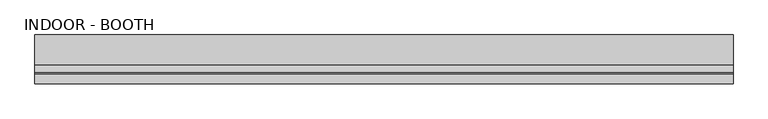
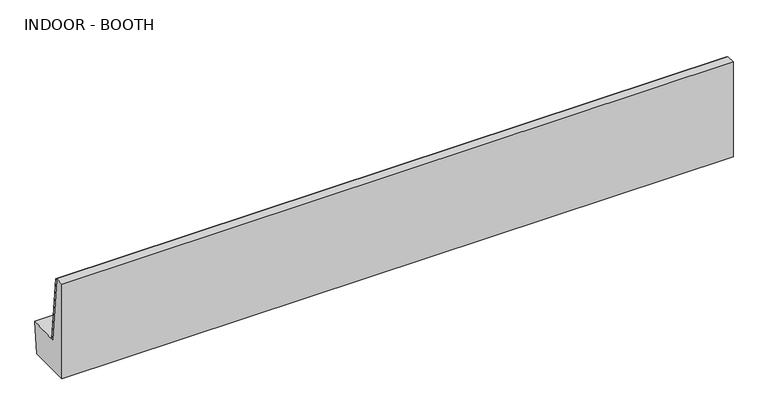
"""IFC4 building model written with IfcOpenShell, lengths in millimetres: furniture geometry, OD_CW_Booth : INDOOR - BOOTH."""

import ifcopenshell
import ifcopenshell.guid

model = None  # the IFC model being written
_history = None  # IfcOwnerHistory: only IFC2X3 demands one
_inside = {}  # id of a spatial element -> (the spatial element, [elements in it])
_under = {}  # id of a project, library or spatial element -> (it, [spatial elements below it])
_declared = {}  # id of a project -> (the project, [libraries it declares])
_typed = {}  # id of a type object -> (the type object, [elements of that type])
_made_of = {}  # id of a material, layer set ... -> (it, [elements and type objects made of it])


def new_model(schema):
    """Start an empty IFC model of exactly this schema.

    Asked for "IFC4X3", IfcOpenShell would pick the latest addendum, in which some entities
    have other attributes; the version numbers below select the first issue.
    IFC2X3 requires an IfcOwnerHistory on every rooted entity: one is made here for all.
    """
    global model, _history
    if schema == "IFC4X3":
        model = ifcopenshell.file(schema_version=(4, 3, 0, 0))
    else:
        model = ifcopenshell.file(schema=schema)
    _inside.clear()
    _under.clear()
    _declared.clear()
    _typed.clear()
    _made_of.clear()
    _history = None
    if model.schema == "IFC2X3":
        org = make("IfcOrganization", Name="unknown")
        user = make(
            "IfcPersonAndOrganization",
            ThePerson=make("IfcPerson", FamilyName="unknown"),
            TheOrganization=org,
        )
        app = make(
            "IfcApplication",
            ApplicationDeveloper=org,
            Version="unknown",
            ApplicationFullName="unknown",
            ApplicationIdentifier="unknown",
        )
        _history = make(
            "IfcOwnerHistory",
            OwningUser=user,
            OwningApplication=app,
            ChangeAction="ADDED",
            CreationDate=0,
        )
    return model


def make(cls, **values):
    """One entity of the class cls with the attributes given. An attribute that is None is left unset."""
    return model.create_entity(
        cls, **{name: value for name, value in values.items() if value is not None}
    )


def rooted(cls, **values):
    """An entity with a GlobalId (a new one), such as an element, a storey or a relation."""
    return make(cls, GlobalId=ifcopenshell.guid.new(), OwnerHistory=_history, **values)


def si_unit(unit_type, name, prefix=None):
    """IfcSIUnit, for example si_unit("LENGTHUNIT", "METRE", prefix="MILLI")."""
    return make("IfcSIUnit", UnitType=unit_type, Prefix=prefix, Name=name)


def assignment(units):
    """IfcUnitAssignment: the units of a project."""
    return None if units is None else make("IfcUnitAssignment", Units=units)


def point(xyz):
    """IfcCartesianPoint."""
    return None if xyz is None else make("IfcCartesianPoint", Coordinates=xyz)


def direction(xyz):
    """IfcDirection."""
    return None if xyz is None else make("IfcDirection", DirectionRatios=xyz)


def frame(location, z_axis=None, x_axis=None):
    """IfcAxis2Placement3D, a coordinate frame: its origin and axes. An axis left out is left unset."""
    return make(
        "IfcAxis2Placement3D",
        Location=point(location),
        Axis=direction(z_axis),
        RefDirection=direction(x_axis),
    )


def origin():
    """The frame at (0, 0, 0) with its axes left unset."""
    return frame((0.0, 0.0, 0.0))


def place(relative_to, where):
    """IfcLocalPlacement: puts the frame where relative to a parent placement (None: the world)."""
    return make(
        "IfcLocalPlacement", PlacementRelTo=relative_to, RelativePlacement=where
    )


def context(
    kind, dimensions, precision=None, world=None, true_north=None, identifier=None
):
    """IfcGeometricRepresentationContext, for example the 3D "Model" context."""
    return make(
        "IfcGeometricRepresentationContext",
        ContextIdentifier=identifier,
        ContextType=kind,
        CoordinateSpaceDimension=dimensions,
        Precision=precision,
        WorldCoordinateSystem=world,
        TrueNorth=true_north,
    )


def project(units=None, contexts=None):
    """IfcProject with its units and contexts."""
    return rooted(
        "IfcProject",
        Name="project",
        RepresentationContexts=contexts,
        UnitsInContext=assignment(units),
    )


def spatial(cls, under=None, at=None, **own):
    """A site, building, storey or space (cls), placed at a placement, below another one or the project."""
    s = rooted(cls, ObjectPlacement=at, **own)
    if under is not None:
        _under.setdefault(under.id(), (under, []))[1].append(s)
    return s


def polyline(points):
    """IfcPolyline through the points."""
    return make("IfcPolyline", Points=[point(p) for p in points])


def outline(outer, holes=None, kind="AREA"):
    """IfcArbitraryClosedProfileDef: a profile drawn as a closed curve; with holes, ...WithVoids."""
    if holes is None:
        return make("IfcArbitraryClosedProfileDef", ProfileType=kind, OuterCurve=outer)
    return make(
        "IfcArbitraryProfileDefWithVoids",
        ProfileType=kind,
        OuterCurve=outer,
        InnerCurves=holes,
    )


def extrude(swept, where, along, depth):
    """IfcExtrudedAreaSolid: the profile swept, set in the frame where, extruded along a direction by depth."""
    return make(
        "IfcExtrudedAreaSolid",
        SweptArea=swept,
        Position=where,
        ExtrudedDirection=direction(along),
        Depth=depth,
    )


def shape(context_of_items, identifier, shape_type, items):
    """IfcShapeRepresentation: the items that make up one representation, for example the "Body"."""
    return make(
        "IfcShapeRepresentation",
        ContextOfItems=context_of_items,
        RepresentationIdentifier=identifier,
        RepresentationType=shape_type,
        Items=items,
    )


def source(mapping_origin, context_of_items, identifier, shape_type, items):
    """IfcRepresentationMap: a shape defined once, which mapped items show again and again."""
    return make(
        "IfcRepresentationMap",
        MappingOrigin=mapping_origin,
        MappedRepresentation=shape(context_of_items, identifier, shape_type, items),
    )


def transform(
    local_origin,
    x_axis=None,
    y_axis=None,
    z_axis=None,
    scale=None,
    scale2=None,
    scale3=None,
    uniform=True,
):
    """IfcCartesianTransformationOperator3D, or its non-uniform kind. x_axis, y_axis, z_axis: its Axis1, 2, 3."""
    if uniform:
        return make(
            "IfcCartesianTransformationOperator3D",
            Axis1=direction(x_axis),
            Axis2=direction(y_axis),
            LocalOrigin=point(local_origin),
            Scale=scale,
            Axis3=direction(z_axis),
        )
    return make(
        "IfcCartesianTransformationOperator3DnonUniform",
        Axis1=direction(x_axis),
        Axis2=direction(y_axis),
        LocalOrigin=point(local_origin),
        Scale=scale,
        Axis3=direction(z_axis),
        Scale2=scale2,
        Scale3=scale3,
    )


def mapped(mapping_source, mapping_target):
    """IfcMappedItem: shows the shape of a source again, moved by a transform."""
    return make(
        "IfcMappedItem", MappingSource=mapping_source, MappingTarget=mapping_target
    )


def made_of(thing, what):
    """Note that an element or type object is made of a material, layer set ...; save() writes the relation."""
    if what is not None:
        _made_of.setdefault(what.id(), (what, []))[1].append(thing)
    return thing


def element(
    cls,
    number,
    at=None,
    inside=None,
    cuts=None,
    type_object=None,
    material=None,
    context=None,
    identifier="Body",
    shape_type=None,
    held_by="IfcProductDefinitionShape",
    body=None,
    shapes=None,
    **own,
):
    """One element of the class cls, such as IfcWall. Its Tag is "e" and its number.

    at: its placement. inside: the storey or other place that contains it. cuts: it is an
    opening in that element (IfcRelVoidsElement). A single representation is given by context,
    identifier, shape_type and body (its items); several are given by shapes. held_by: the class
    of the entity that holds the representations. save() writes the other relations.
    """
    e = rooted(cls, Tag="e%d" % number, ObjectPlacement=at, **own)
    if body is not None:
        shapes = [shape(context, identifier, shape_type, body)]
    if shapes is not None:
        e.Representation = make(held_by, Representations=shapes)
    if inside is not None:
        _inside.setdefault(inside.id(), (inside, []))[1].append(e)
    if cuts is not None:
        rooted(
            "IfcRelVoidsElement", RelatingBuildingElement=cuts, RelatedOpeningElement=e
        )
    if type_object is not None:
        _typed.setdefault(type_object.id(), (type_object, []))[1].append(e)
    return made_of(e, material)


def aggregate(whole, parts):
    """IfcRelAggregates: a whole, such as a stair, and the parts it consists of."""
    return rooted("IfcRelAggregates", RelatingObject=whole, RelatedObjects=parts)


def save(model, path):
    """Write the relations noted so far, then the file.

    IfcRelAggregates (storeys below a building ...), IfcRelContainedInSpatialStructure (elements
    in a storey), IfcRelDefinesByType, IfcRelAssociatesMaterial and IfcRelDeclares: one each for
    every whole, place, type object, material and project.
    """
    for whole, parts in _under.values():
        aggregate(whole, parts)
    for where, things in _inside.values():
        rooted(
            "IfcRelContainedInSpatialStructure",
            RelatedElements=things,
            RelatingStructure=where,
        )
    for kind, things in _typed.values():
        rooted("IfcRelDefinesByType", RelatedObjects=things, RelatingType=kind)
    for what, things in _made_of.values():
        rooted("IfcRelAssociatesMaterial", RelatedObjects=things, RelatingMaterial=what)
    for by, libraries in _declared.values():
        rooted("IfcRelDeclares", RelatingContext=by, RelatedDefinitions=libraries)
    model.write(path)


def indoor_booth_a2b8d8e1(model_context):
    return source(origin(), model_context, "Body", "SweptSolid", [
        extrude(outline(polyline([(0.0, -9357.0837874), (0.0, 0.0), (25.4, 0.0), (25.4, -9357.0837874), (0.0, -9357.0837874)])), frame((9375.8214923, -358.2049359, 438.8309433), z_axis=(0.0, -0.10452846326765197, 0.9945218953682735), x_axis=(0.0, -0.9945218953682735, -0.10452846326765197)), (0.0, 0.0, 1.0), 944.7333479),
        extrude(outline(polyline([(-609.6, 1397.0), (-484.4524721, 1397.0), (-382.9385128, 431.1591941), (43.0849153, 453.4861359), (3.4100193, 0.0), (-609.6, 0.0), (-609.6, 1397.0)])), frame((18.7377049, 0.0, 0.0), z_axis=(1.0, 0.0, 0.0), x_axis=(0.0, 1.0, 0.0)), (0.0, 0.0, 1.0), 9357.0837874),
    ])


if __name__ == "__main__":
    model = new_model("IFC4")
    model_context = context("Model", 3, world=origin())
    ifc_project = project(units=[si_unit("LENGTHUNIT", "METRE", prefix="MILLI")], contexts=[model_context])
    site = spatial("IfcSite", under=ifc_project)
    building = spatial("IfcBuilding", under=site)
    placement = place(None, origin())
    indoor_booth_shape = indoor_booth_a2b8d8e1(model_context)
    element("IfcFurniture", 1, ObjectType="OD_CW_Booth : INDOOR - BOOTH", at=placement, inside=building, context=model_context, shape_type="MappedRepresentation", body=[
        mapped(indoor_booth_shape, transform((0.0, 0.0, 0.0), x_axis=(1.0, 0.0, 0.0), y_axis=(0.0, 1.0, 0.0), z_axis=(0.0, 0.0, 1.0))),
    ])
    save(model, "model.ifc")

# Revit data of these elements
# Type "OD_CW_Booth : INDOOR - BOOTH"
#   Type Mark = "TYPE - INDOOR - BOOTH"
#   Width = 4' - 0"
#   OD_CW_Width [instance default] = 2' - 10"
#   OD_CW_Length [instance default] = 26' - 1 83/256"
#   OD_CW_Height [instance default] = 2' - 3"
#   Height = 3' - 0"
#   Depth = 2' - 0"
#   Seating Count [instance default] = 10
#   Seating Count [instance default] = 10
#   back = Casework-oakfire
#   OD_CW_Material_Front Panel [instance default] = none
#   OD_CW_Material_Body [instance default] = none
# Element 1 (IfcFurniture, "OD_CW_Booth : INDOOR - BOOTH")
#   OD_CW_Length = 30' - 8.38913"
#   Seating Count = 11
#   OD_CW_Material_Body = WOOD-OAKFIRE
#   Materials on its faces: "WOOD-OAKFIRE", "Casework-oakfire"
# Materials
#   "Casework-oakfire": class "Miscellaneous", colour RGB 164 164 164, transparency 0, Cost = 0
#   "WOOD-OAKFIRE": class "Wood", colour RGB 198 202 183, transparency 0, Description = "Generic wood", Cost = 0
